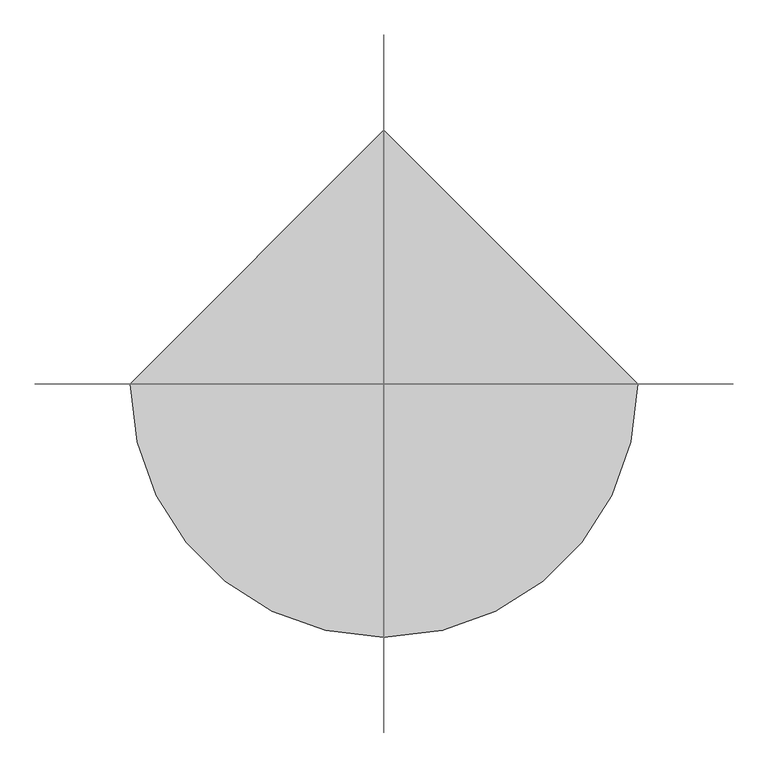
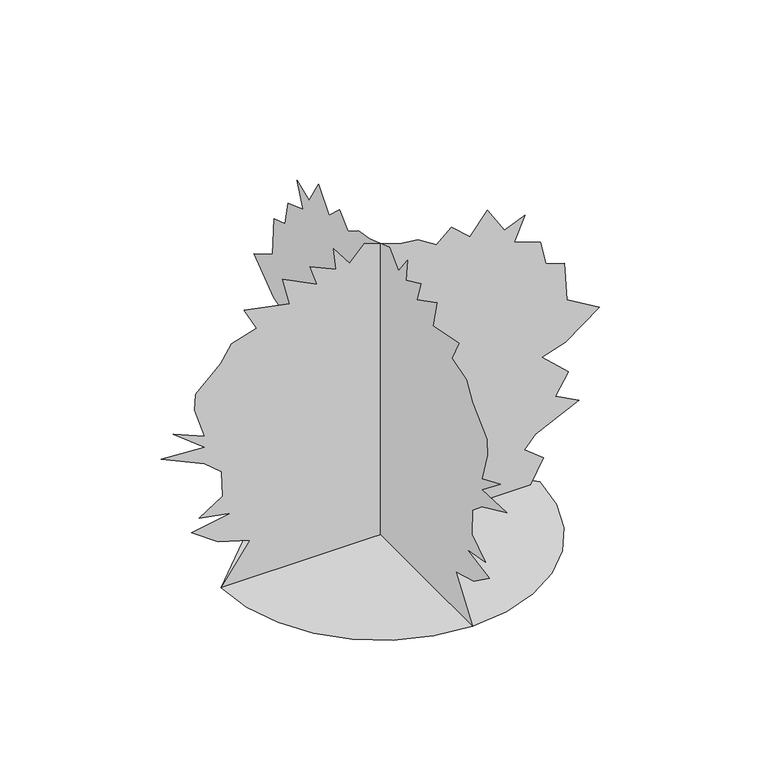
"""IFC4 building model written with IfcOpenShell, lengths in millimetres: proxy geometry, oleander 26757 : oleander 26757."""

from ifc_helpers import new_model, si_unit, origin, place, context, project, spatial, triangles, source, transform, mapped, element, save


def entourage_e0fef716(model_context):
    return source(origin(), model_context, "Body", "Tessellation", [
        triangles([(-812.5409557, 0.0, 3.62e-05), (-791.0601448, -186.180478, 3.62e-05), (-729.881757, -357.1570149, 3.62e-05), (-633.9078186, -508.0330527, 3.62e-05), (-508.0330527, -633.9078186, 3.62e-05), (-357.1570149, -729.881757, 3.62e-05), (-186.180478, -791.0601448, 3.62e-05), (3.55e-05, -812.5409557, 3.62e-05), (186.180478, -791.0601448, 3.62e-05), (357.1570149, -729.881757, 3.62e-05), (508.0330527, -633.9078186, 3.62e-05), (633.9078186, -508.0330527, 3.62e-05), (729.881757, -357.1570149, 3.62e-05), (791.0601448, -186.180478, 3.62e-05), (812.5409557, 7.1e-05, 3.62e-05), (-0.0001066, 812.5409557, 3.62e-05), (-0.0042747, -811.2988804, 0.0001209), (-0.0042708, -665.7314575, 204.5081021), (-0.004267, -827.900338, 251.4511125), (-0.004262, -964.4608978, 349.6056227), (-0.004264, -763.884696, 383.7457626), (-0.0042607, -926.0535765, 413.6186849), (-0.0042602, -806.5618149, 490.4333639), (-0.0042562, -810.8289963, 622.7267424), (-0.0042527, -896.1806179, 695.2767471), (-0.0042464, -1118.0927994, 797.697167), (-0.0042501, -896.1806179, 784.8930794), (-0.0042438, -1058.3468822, 912.9192038), (-0.0042483, -896.1806179, 844.6389238), (-0.0042428, -947.3895561, 1002.5380068), (-0.0042404, -943.1223747, 1087.8896284), (-0.0042387, -815.0961777, 1207.38139), (-0.0042368, -759.6175146, 1297.000193), (-0.0042376, -631.5913176, 1335.4075871), (-0.0042331, -695.6044161, 1454.899276), (-0.0042379, -465.1578355, 1407.9550484), (-0.0042331, -499.2979754, 1553.0525871), (-0.0042384, -324.3300579, 1463.4337841), (-0.0042347, -358.4701979, 1570.1213127), (-0.0042384, -226.175584, 1510.3755409), (-0.0042348, -238.9782001, 1625.6000484), (-0.0042392, -157.8947954, 1518.9123745), (-0.0042379, -81.0790899, 1599.9943439), (-0.0042425, 98.1577985, 1535.9812454), (-0.0042443, 192.0433106, 1523.1795559), (-0.0042475, 285.9303487, 1463.4337841), (-0.0042466, 362.7450459, 1531.714064), (-0.0042505, 456.6310667, 1446.3624424), (-0.0042486, 546.2498697, 1557.3197685), (-0.0042539, 631.6014914, 1420.7592087), (-0.0042542, 738.2890926, 1463.4337841), (-0.0042571, 682.8104296, 1339.6747684), (-0.0042604, 815.1063515, 1292.7305408), (-0.0042647, 844.9767666, 1164.7043438), (-0.004267, 938.862751, 1134.8313852), (-0.0042731, 951.6669113, 934.2577269), (-0.0042786, 1118.1004297, 836.104561), (-0.0042798, 943.1324759, 708.078364), (-0.0042791, 823.6407143, 669.6710426), (-0.004285, 960.2012741, 541.6448456), (-0.0042871, 891.9209942, 434.9547009), (-0.0042908, 1011.4127558, 370.9416023), (-0.0042907, 789.5005743, 264.2539829), (-0.0042918, 734.0219112, 200.2406482), (-0.0042955, 832.1751497, 123.4246974), (-0.0042982, 766.4170996, 0.0205859), (-811.3090542, 0.0043453, 0.0), (-665.7416313, 0.0043331, 204.5081021), (-827.9079683, 0.0043303, 251.4511125), (-964.4685282, 0.0043245, 349.6056227), (-763.8948698, 0.0043224, 383.7457626), (-926.0611341, 0.0043206, 413.6186849), (-806.5693726, 0.0043161, 490.4333639), (-810.8366266, 0.0043082, 622.7267424), (-896.1882483, 0.0043039, 695.2742037), (-1118.1004297, 0.0042978, 797.697167), (-896.1882483, 0.0042985, 784.8930794), (-1058.3545126, 0.0042909, 912.9192038), (-896.1882483, 0.004295, 844.6389238), (-947.3997299, 0.0042855, 1002.5380068), (-943.1299324, 0.0042805, 1087.8896284), (-815.1063515, 0.0042733, 1207.38139), (-759.6276884, 0.004268, 1297.000193), (-631.6014914, 0.0042657, 1335.4075871), (-695.6145899, 0.0042586, 1454.899276), (-465.1654658, 0.0042614, 1407.9550484), (-499.3056058, 0.0042527, 1553.0525871), (-324.3376883, 0.0042581, 1463.4337841), (-358.4778282, 0.0042517, 1570.1213127), (-226.1839592, 0.0042553, 1510.3755409), (-238.9868297, 0.0042484, 1625.6000484), (-157.903425, 0.0042548, 1518.9123745), (-81.0877285, 0.0042499, 1599.9943439), (98.1491599, 0.0042537, 1535.9812454), (192.034681, 0.0042545, 1523.1795559), (285.9201931, 0.0042581, 1463.4337841), (362.7374156, 0.004254, 1531.714064), (456.6234364, 0.0042591, 1446.3624424), (546.2422394, 0.0042525, 1557.3197685), (631.5913176, 0.0042606, 1420.7565926), (738.281535, 0.0042581, 1463.4337841), (682.8027992, 0.0042654, 1339.6747684), (815.0961777, 0.0042682, 1292.7305408), (844.9691362, 0.0042759, 1164.7043438), (938.8551207, 0.0042777, 1134.8313852), (951.6567375, 0.0042896, 934.2577269), (1118.0927994, 0.0042955, 836.104561), (943.1223747, 0.0043031, 708.078364), (823.6306131, 0.0043054, 669.6710426), (960.1937164, 0.004313, 541.6448456), (891.9134365, 0.0043194, 434.9547009), (1011.4026546, 0.0043232, 370.9416023), (789.4904732, 0.0043296, 264.2539829), (734.0142809, 0.0043334, 200.2403938), (832.1675194, 0.0043379, 123.4246974), (766.4094692, 0.0043453, 0.020512)], [[15, 16, 1], [14, 15, 1], [14, 1, 2], [13, 14, 2], [13, 2, 3], [13, 3, 4], [12, 13, 4], [11, 12, 4], [11, 4, 5], [11, 5, 6], [11, 6, 7], [11, 7, 8], [11, 8, 9], [11, 9, 10], [27, 28, 29], [25, 26, 27], [40, 41, 42], [21, 22, 23], [50, 51, 52], [19, 20, 21], [38, 39, 40], [36, 37, 38], [34, 35, 36], [61, 62, 63], [66, 17, 18], [56, 57, 58], [48, 49, 50], [18, 19, 21], [46, 47, 48], [64, 65, 66], [59, 60, 61], [56, 58, 59], [54, 55, 56], [42, 43, 44], [52, 53, 54], [54, 56, 59], [24, 25, 27], [48, 50, 52], [59, 61, 63], [52, 54, 59], [48, 52, 59], [46, 48, 59], [66, 18, 21], [30, 31, 32], [29, 30, 32], [66, 21, 23], [66, 23, 24], [64, 66, 24], [63, 64, 24], [59, 63, 24], [46, 59, 24], [45, 46, 24], [44, 45, 24], [42, 44, 24], [40, 42, 24], [38, 40, 24], [36, 38, 24], [34, 36, 24], [34, 24, 27], [34, 27, 29], [34, 29, 32], [33, 34, 32], [77, 78, 79], [75, 76, 77], [90, 91, 92], [71, 72, 73], [100, 101, 102], [69, 70, 71], [88, 89, 90], [86, 87, 88], [84, 85, 86], [111, 112, 113], [116, 67, 68], [106, 107, 108], [98, 99, 100], [68, 69, 71], [96, 97, 98], [114, 115, 116], [109, 110, 111], [106, 108, 109], [104, 105, 106], [92, 93, 94], [102, 103, 104], [104, 106, 109], [74, 75, 77], [98, 100, 102], [109, 111, 113], [102, 104, 109], [98, 102, 109], [96, 98, 109], [116, 68, 71], [80, 81, 82], [79, 80, 82], [116, 71, 73], [116, 73, 74], [114, 116, 74], [113, 114, 74], [109, 113, 74], [96, 109, 74], [95, 96, 74], [94, 95, 74], [92, 94, 74], [90, 92, 74], [88, 90, 74], [86, 88, 74], [84, 86, 74], [84, 74, 77], [84, 77, 79], [84, 79, 82], [83, 84, 82]], closed=False),
    ])


if __name__ == "__main__":
    model = new_model("IFC4")
    model_context = context("Model", 3, world=origin())
    ifc_project = project(units=[si_unit("LENGTHUNIT", "METRE", prefix="MILLI")], contexts=[model_context])
    site = spatial("IfcSite", under=ifc_project)
    building = spatial("IfcBuilding", under=site)
    placement = place(None, origin())
    entourage_shape = entourage_e0fef716(model_context)
    element("IfcBuildingElementProxy", 1, Name="oleander 26757 : oleander 26757", ObjectType="oleander 26757 : oleander 26757", at=placement, inside=building, context=model_context, shape_type="MappedRepresentation", body=[
        mapped(entourage_shape, transform((0.0, 0.0, 0.0), x_axis=(1.0, 0.0, 0.0), y_axis=(0.0, 1.0, 0.0), z_axis=(0.0, 0.0, 1.0))),
    ])
    save(model, "model.ifc")

# Revit data of these elements
# Type "oleander 26757 : oleander 26757"
#   built-in parameter 1005195 = "RPC-16-G3GJ-A6PX-PK1P-U000-ST1L-LVER-AU"
#   Height = 0
